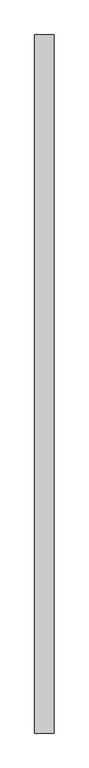
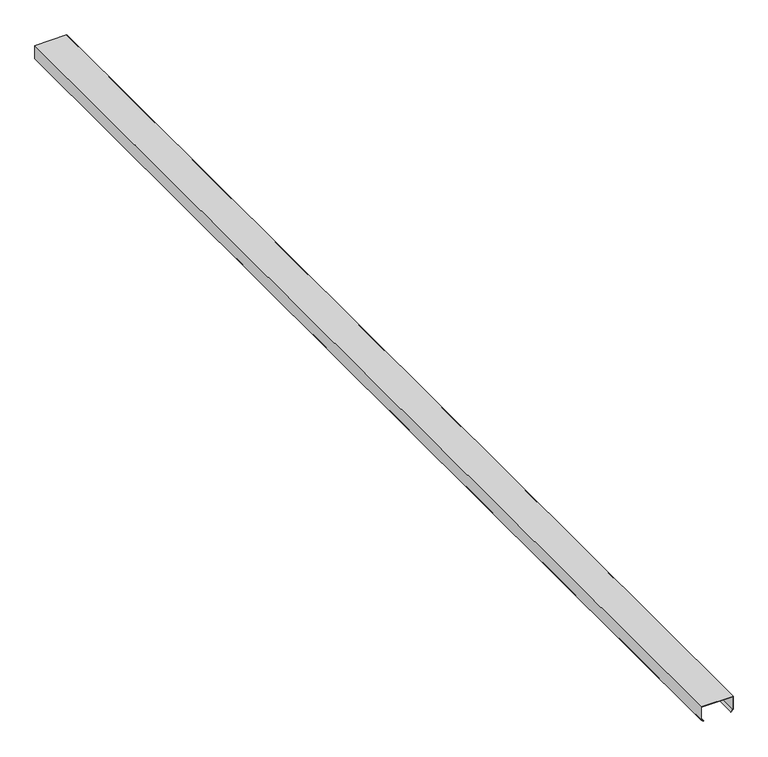
"""IFC4 building model written with IfcOpenShell, lengths in millimetres: proxy geometry, Generic Models 7:Generic Models 1:1:Generic Models 1:1 : Generic Models 7:Generic Models 1:337419:26 : Generic Models 7:Generic Models 1:1:Generic Models 1:1 : Generic Models 7:Generic Models 1:337419:306201."""

import ifcopenshell
import ifcopenshell.guid

model = None  # the IFC model being written
_history = None  # IfcOwnerHistory: only IFC2X3 demands one
_inside = {}  # id of a spatial element -> (the spatial element, [elements in it])
_under = {}  # id of a project, library or spatial element -> (it, [spatial elements below it])
_declared = {}  # id of a project -> (the project, [libraries it declares])
_typed = {}  # id of a type object -> (the type object, [elements of that type])
_made_of = {}  # id of a material, layer set ... -> (it, [elements and type objects made of it])


def new_model(schema):
    """Start an empty IFC model of exactly this schema.

    Asked for "IFC4X3", IfcOpenShell would pick the latest addendum, in which some entities
    have other attributes; the version numbers below select the first issue.
    IFC2X3 requires an IfcOwnerHistory on every rooted entity: one is made here for all.
    """
    global model, _history
    if schema == "IFC4X3":
        model = ifcopenshell.file(schema_version=(4, 3, 0, 0))
    else:
        model = ifcopenshell.file(schema=schema)
    _inside.clear()
    _under.clear()
    _declared.clear()
    _typed.clear()
    _made_of.clear()
    _history = None
    if model.schema == "IFC2X3":
        org = make("IfcOrganization", Name="unknown")
        user = make(
            "IfcPersonAndOrganization",
            ThePerson=make("IfcPerson", FamilyName="unknown"),
            TheOrganization=org,
        )
        app = make(
            "IfcApplication",
            ApplicationDeveloper=org,
            Version="unknown",
            ApplicationFullName="unknown",
            ApplicationIdentifier="unknown",
        )
        _history = make(
            "IfcOwnerHistory",
            OwningUser=user,
            OwningApplication=app,
            ChangeAction="ADDED",
            CreationDate=0,
        )
    return model


def make(cls, **values):
    """One entity of the class cls with the attributes given. An attribute that is None is left unset."""
    return model.create_entity(
        cls, **{name: value for name, value in values.items() if value is not None}
    )


def rooted(cls, **values):
    """An entity with a GlobalId (a new one), such as an element, a storey or a relation."""
    return make(cls, GlobalId=ifcopenshell.guid.new(), OwnerHistory=_history, **values)


def si_unit(unit_type, name, prefix=None):
    """IfcSIUnit, for example si_unit("LENGTHUNIT", "METRE", prefix="MILLI")."""
    return make("IfcSIUnit", UnitType=unit_type, Prefix=prefix, Name=name)


def assignment(units):
    """IfcUnitAssignment: the units of a project."""
    return None if units is None else make("IfcUnitAssignment", Units=units)


def point(xyz):
    """IfcCartesianPoint."""
    return None if xyz is None else make("IfcCartesianPoint", Coordinates=xyz)


def direction(xyz):
    """IfcDirection."""
    return None if xyz is None else make("IfcDirection", DirectionRatios=xyz)


def frame(location, z_axis=None, x_axis=None):
    """IfcAxis2Placement3D, a coordinate frame: its origin and axes. An axis left out is left unset."""
    return make(
        "IfcAxis2Placement3D",
        Location=point(location),
        Axis=direction(z_axis),
        RefDirection=direction(x_axis),
    )


def origin():
    """The frame at (0, 0, 0) with its axes left unset."""
    return frame((0.0, 0.0, 0.0))


def place(relative_to, where):
    """IfcLocalPlacement: puts the frame where relative to a parent placement (None: the world)."""
    return make(
        "IfcLocalPlacement", PlacementRelTo=relative_to, RelativePlacement=where
    )


def context(
    kind, dimensions, precision=None, world=None, true_north=None, identifier=None
):
    """IfcGeometricRepresentationContext, for example the 3D "Model" context."""
    return make(
        "IfcGeometricRepresentationContext",
        ContextIdentifier=identifier,
        ContextType=kind,
        CoordinateSpaceDimension=dimensions,
        Precision=precision,
        WorldCoordinateSystem=world,
        TrueNorth=true_north,
    )


def project(units=None, contexts=None):
    """IfcProject with its units and contexts."""
    return rooted(
        "IfcProject",
        Name="project",
        RepresentationContexts=contexts,
        UnitsInContext=assignment(units),
    )


def spatial(cls, under=None, at=None, **own):
    """A site, building, storey or space (cls), placed at a placement, below another one or the project."""
    s = rooted(cls, ObjectPlacement=at, **own)
    if under is not None:
        _under.setdefault(under.id(), (under, []))[1].append(s)
    return s


def polyline(points):
    """IfcPolyline through the points."""
    return make("IfcPolyline", Points=[point(p) for p in points])


def outline(outer, holes=None, kind="AREA"):
    """IfcArbitraryClosedProfileDef: a profile drawn as a closed curve; with holes, ...WithVoids."""
    if holes is None:
        return make("IfcArbitraryClosedProfileDef", ProfileType=kind, OuterCurve=outer)
    return make(
        "IfcArbitraryProfileDefWithVoids",
        ProfileType=kind,
        OuterCurve=outer,
        InnerCurves=holes,
    )


def extrude(swept, where, along, depth):
    """IfcExtrudedAreaSolid: the profile swept, set in the frame where, extruded along a direction by depth."""
    return make(
        "IfcExtrudedAreaSolid",
        SweptArea=swept,
        Position=where,
        ExtrudedDirection=direction(along),
        Depth=depth,
    )


def shape(context_of_items, identifier, shape_type, items):
    """IfcShapeRepresentation: the items that make up one representation, for example the "Body"."""
    return make(
        "IfcShapeRepresentation",
        ContextOfItems=context_of_items,
        RepresentationIdentifier=identifier,
        RepresentationType=shape_type,
        Items=items,
    )


def source(mapping_origin, context_of_items, identifier, shape_type, items):
    """IfcRepresentationMap: a shape defined once, which mapped items show again and again."""
    return make(
        "IfcRepresentationMap",
        MappingOrigin=mapping_origin,
        MappedRepresentation=shape(context_of_items, identifier, shape_type, items),
    )


def transform(
    local_origin,
    x_axis=None,
    y_axis=None,
    z_axis=None,
    scale=None,
    scale2=None,
    scale3=None,
    uniform=True,
):
    """IfcCartesianTransformationOperator3D, or its non-uniform kind. x_axis, y_axis, z_axis: its Axis1, 2, 3."""
    if uniform:
        return make(
            "IfcCartesianTransformationOperator3D",
            Axis1=direction(x_axis),
            Axis2=direction(y_axis),
            LocalOrigin=point(local_origin),
            Scale=scale,
            Axis3=direction(z_axis),
        )
    return make(
        "IfcCartesianTransformationOperator3DnonUniform",
        Axis1=direction(x_axis),
        Axis2=direction(y_axis),
        LocalOrigin=point(local_origin),
        Scale=scale,
        Axis3=direction(z_axis),
        Scale2=scale2,
        Scale3=scale3,
    )


def mapped(mapping_source, mapping_target):
    """IfcMappedItem: shows the shape of a source again, moved by a transform."""
    return make(
        "IfcMappedItem", MappingSource=mapping_source, MappingTarget=mapping_target
    )


def made_of(thing, what):
    """Note that an element or type object is made of a material, layer set ...; save() writes the relation."""
    if what is not None:
        _made_of.setdefault(what.id(), (what, []))[1].append(thing)
    return thing


def element(
    cls,
    number,
    at=None,
    inside=None,
    cuts=None,
    type_object=None,
    material=None,
    context=None,
    identifier="Body",
    shape_type=None,
    held_by="IfcProductDefinitionShape",
    body=None,
    shapes=None,
    **own,
):
    """One element of the class cls, such as IfcWall. Its Tag is "e" and its number.

    at: its placement. inside: the storey or other place that contains it. cuts: it is an
    opening in that element (IfcRelVoidsElement). A single representation is given by context,
    identifier, shape_type and body (its items); several are given by shapes. held_by: the class
    of the entity that holds the representations. save() writes the other relations.
    """
    e = rooted(cls, Tag="e%d" % number, ObjectPlacement=at, **own)
    if body is not None:
        shapes = [shape(context, identifier, shape_type, body)]
    if shapes is not None:
        e.Representation = make(held_by, Representations=shapes)
    if inside is not None:
        _inside.setdefault(inside.id(), (inside, []))[1].append(e)
    if cuts is not None:
        rooted(
            "IfcRelVoidsElement", RelatingBuildingElement=cuts, RelatedOpeningElement=e
        )
    if type_object is not None:
        _typed.setdefault(type_object.id(), (type_object, []))[1].append(e)
    return made_of(e, material)


def aggregate(whole, parts):
    """IfcRelAggregates: a whole, such as a stair, and the parts it consists of."""
    return rooted("IfcRelAggregates", RelatingObject=whole, RelatedObjects=parts)


def save(model, path):
    """Write the relations noted so far, then the file.

    IfcRelAggregates (storeys below a building ...), IfcRelContainedInSpatialStructure (elements
    in a storey), IfcRelDefinesByType, IfcRelAssociatesMaterial and IfcRelDeclares: one each for
    every whole, place, type object, material and project.
    """
    for whole, parts in _under.values():
        aggregate(whole, parts)
    for where, things in _inside.values():
        rooted(
            "IfcRelContainedInSpatialStructure",
            RelatedElements=things,
            RelatingStructure=where,
        )
    for kind, things in _typed.values():
        rooted("IfcRelDefinesByType", RelatedObjects=things, RelatingType=kind)
    for what, things in _made_of.values():
        rooted("IfcRelAssociatesMaterial", RelatedObjects=things, RelatingMaterial=what)
    for by, libraries in _declared.values():
        rooted("IfcRelDeclares", RelatingContext=by, RelatedDefinitions=libraries)
    model.write(path)


def generic_models_3bf9028a(model_context):
    return source(origin(), model_context, "Body", "SweptSolid", [
        extrude(outline(polyline([(4243.1890625, 560556.1617239), (4243.1890625, 560352.9617239), (4154.2890625, 560352.9617239), (4142.0439586, 560367.5548705), (4144.1721258, 560369.3406148), (4155.5845235, 560355.7398489), (4240.4109375, 560355.7398489), (4240.4109375, 560553.3835989), (4155.5845235, 560553.3835989), (4144.1721258, 560539.7828329), (4142.0439586, 560541.5685772), (4154.2890625, 560556.1617239), (4243.1890625, 560556.1617239)])), frame((0.0, -579000.6913841, 0.0), z_axis=(0.0, 1.0, 0.0), x_axis=(0.0, 0.0, 1.0)), (0.0, 0.0, 1.0), 7315.2),
    ])


if __name__ == "__main__":
    model = new_model("IFC4")
    model_context = context("Model", 3, world=origin())
    ifc_project = project(units=[si_unit("LENGTHUNIT", "METRE", prefix="MILLI")], contexts=[model_context])
    site = spatial("IfcSite", under=ifc_project)
    building = spatial("IfcBuilding", under=site)
    placement = place(None, origin())
    generic_models_shape = generic_models_3bf9028a(model_context)
    element("IfcBuildingElementProxy", 1, Name="Generic Models 7:Generic Models 1:1:Generic Models 1:1 : Generic Models 7:Generic Models 1:337419:26 : Generic Models 7:Generic Models 1:1:Generic Models 1:1 : Generic Models 7:Generic Models 1:337419:306201", ObjectType="Generic Models 7:Generic Models 1:1:Generic Models 1:1 : Generic Models 7:Generic Models 1:337419:26 : Generic Models 7:Generic Models 1:1:Generic Models 1:1 : Generic Models 7:Generic Models 1:337419:306201", at=placement, inside=building, context=model_context, shape_type="MappedRepresentation", body=[
        mapped(generic_models_shape, transform((0.0, 0.0, 0.0), x_axis=(1.0, 0.0, 0.0), y_axis=(0.0, 1.0, 0.0), z_axis=(0.0, 0.0, 1.0))),
    ])
    save(model, "model.ifc")

# Revit data of these elements
# Type "Generic Models 7:Generic Models 1:1:Generic Models 1:1 : Generic Models 7:Generic Models 1:337419:26 : Generic Models 7:Generic Models 1:1:Generic Models 1:1 : Generic Models 7:Generic Models 1:337419:306201"
#   NameOverride = "Generic Models 7:Generic Models 1:1:Generic Models 1:1 : Generic Models 7:Generic Models 1:337419:306201"
#   ObjectTypeOverride = "Generic Models 1:1 : Generic Models 7:Generic Models 1:337419"
#   Reference = "Generic Models 1"
#   Tag = "306201"
# Element 1 (IfcBuildingElementProxy, "Generic Models 7:Generic Models 1:1:Generic Models 1:1 : Generic Models 7:Generic Models 1:337419:26 : Generic Models 7:Generic Models 1:1:Generic Models 1:1 : Generic Models 7:Generic Models 1:337419:306201")
#   Materials on its faces: "GALVANIZED 'CEE' SECTION (8.0x3.5C - SEE STRUCT. DWGS)"
# Materials
#   "GALVANIZED 'CEE' SECTION (8.0x3.5C - SEE STRUCT. DWGS)": class "Unassigned", colour RGB 210 209 208, transparency 0, Keynote = "M05121300.02", Cost = 0
